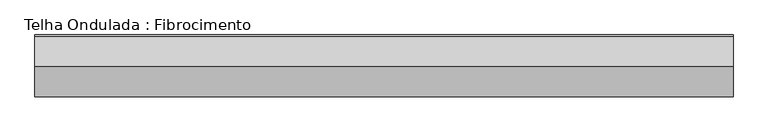
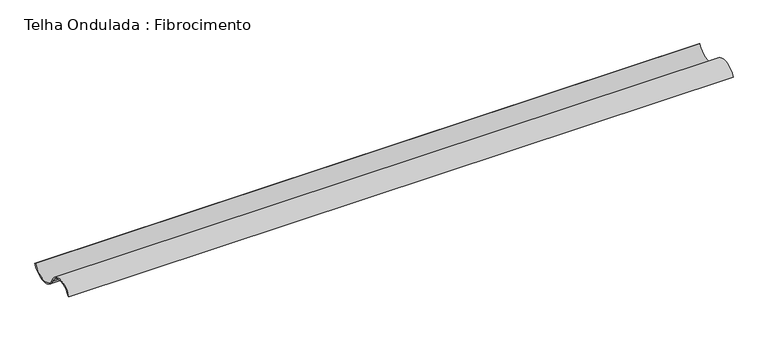
"""IFC4 building model written with IfcOpenShell, lengths in millimetres: beam geometry, Telha Ondulada : Fibrocimento."""

from ifc_helpers import new_model, si_unit, point, frame, frame_2d, origin, place, context, project, spatial, polyline, circle_curve, trimmed, segment, composite_curve, outline, extrude, source, transform, mapped, element, save


def telha_ondulada_fibrocimento_bfc377d9(model_context):
    return source(origin(), model_context, "Body", "SweptSolid", [
        extrude(outline(composite_curve([segment(trimmed(circle_curve(frame_2d((68.3970135, 71.7939461)), 66.7939461), [point((8.3970135, 42.4437972))], [point((128.3970135, 42.4437972))], True, "CARTESIAN"), True, "CONTINUOUS"), segment(polyline([(128.3970135, 42.4437972), (132.8884385, 40.2467307)]), True, "CONTINUOUS"), segment(trimmed(circle_curve(frame_2d((68.3970135, 71.7939461)), 71.7939461), [point((132.8884385, 40.2467307))], [point((3.9055884, 40.2467307))], False, "CARTESIAN"), True, "CONTINUOUS"), segment(trimmed(circle_curve(frame_2d((-51.6029865, 13.0936483)), 61.7939461), [point((3.9055884, 40.2467307))], [point((-107.1115615, 40.2467307))], True, "CARTESIAN"), True, "CONTINUOUS"), segment(polyline([(-107.1115615, 40.2467307), (-111.6029865, 42.4437972)]), True, "CONTINUOUS"), segment(trimmed(circle_curve(frame_2d((-51.6029865, 13.0936483)), 66.7939461), [point((-111.6029865, 42.4437972))], [point((8.3970135, 42.4437972))], False, "CARTESIAN"), True, "CONTINUOUS")], self_intersect=False)), frame((-1382.2210865, 0.0, 0.0), z_axis=(1.0, 0.0, 0.0), x_axis=(0.0, 1.0, 0.0)), (0.0, 0.0, 1.0), 2764.442173),
    ])


if __name__ == "__main__":
    model = new_model("IFC4")
    model_context = context("Model", 3, world=origin())
    ifc_project = project(units=[si_unit("LENGTHUNIT", "METRE", prefix="MILLI")], contexts=[model_context])
    site = spatial("IfcSite", under=ifc_project)
    building = spatial("IfcBuilding", under=site)
    placement = place(None, origin())
    telha_ondulada_fibrocimento_shape = telha_ondulada_fibrocimento_bfc377d9(model_context)
    element("IfcBeam", 1, ObjectType="Telha Ondulada : Fibrocimento", at=placement, inside=building, context=model_context, shape_type="MappedRepresentation", body=[
        mapped(telha_ondulada_fibrocimento_shape, transform((0.0, 0.0, 0.0), x_axis=(1.0, 0.0, 0.0), y_axis=(0.0, 1.0, 0.0), z_axis=(0.0, 0.0, 1.0))),
    ])
    save(model, "model.ifc")

# Revit data of these elements
# Type "Telha Ondulada : Fibrocimento"
#   Description = "TELHA ONDULADA FIBROCIMENTO"
#   Cost = 5
#   Length [instance default] = 1.524 m
#   b = 0.07 m
#   h = 0.16 m
#   Structural Material = .TELHA DE FIBROCIMENTO
#   Assembly Code = ""
# Element 1 (IfcBeam, "Telha Ondulada : Fibrocimento")
#   Materials on its faces: ".TELHA DE FIBROCIMENTO"
# Materials
#   ".TELHA DE FIBROCIMENTO": class "CC_TELHADO", colour RGB 77 77 76, transparency 0, Description = "TELHA ONDULADA FIBROCIMENTO", Cost = 0
